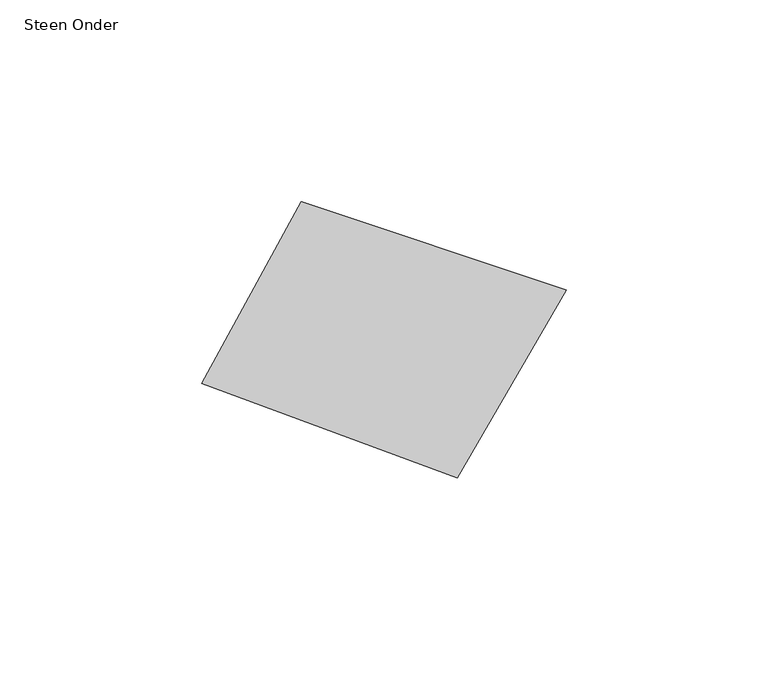
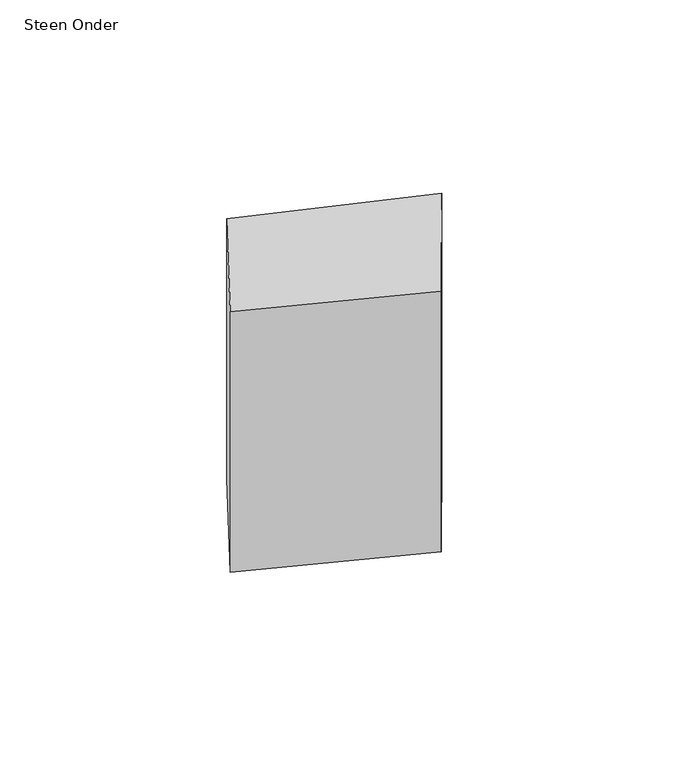
"""IFC4 building model written with IfcOpenShell, lengths in millimetres: proxy geometry, 00_GMA_steen_versie_4 : Steen Onder."""

from ifc_helpers import new_model, si_unit, frame, origin, place, context, project, spatial, polyline, outline, extrude, source, transform, mapped, element, save


def steen_onder_aecb5c40(model_context):
    return source(origin(), model_context, "Body", "SweptSolid", [
        extrude(outline(polyline([(133.5720311, 54.035908), (106.5414453, 7.4740156), (43.3419637, 30.9925765), (67.9706883, 75.9866027), (133.5720311, 54.035908)])), frame((0.0, 0.0, -100.0), z_axis=(0.0, 0.0, 1.0), x_axis=(1.0, 0.0, 0.0)), (0.0, 0.0, 1.0), 100.0),
    ])


if __name__ == "__main__":
    model = new_model("IFC4")
    model_context = context("Model", 3, world=origin())
    ifc_project = project(units=[si_unit("LENGTHUNIT", "METRE", prefix="MILLI")], contexts=[model_context])
    site = spatial("IfcSite", under=ifc_project)
    building = spatial("IfcBuilding", under=site)
    placement = place(None, origin())
    steen_onder_shape = steen_onder_aecb5c40(model_context)
    element("IfcBuildingElementProxy", 1, Name="00_GMA_steen_versie_4 : Steen Onder", ObjectType="00_GMA_steen_versie_4 : Steen Onder", at=placement, inside=building, context=model_context, shape_type="MappedRepresentation", body=[
        mapped(steen_onder_shape, transform((0.0, 0.0, 0.0), x_axis=(1.0, 0.0, 0.0), y_axis=(0.0, 1.0, 0.0), z_axis=(0.0, 0.0, 1.0))),
    ])
    save(model, "model.ifc")

# Revit data of these elements
# Type "00_GMA_steen_versie_4 : Steen Onder"
#   StootVoegHalfBoven [instance default] = 5 mm
#   StootVoegHalf [instance default] = 5 mm
#   StootVoegBreedteOnder = 10 mm
#   StootVoegBreedteBoven = 10 mm
#   Steendikte = 100 mm
#   LintVoegOnderHalf = 0 mm
#   LintVoegOnder = 0 mm
#   LintVoegBovenHalf = 5 mm
#   LintVoegBoven = 10 mm
#   materiaal = none
#   MateriaalVoeg = none
#   Default Elevation = 0
